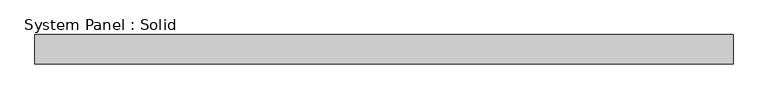
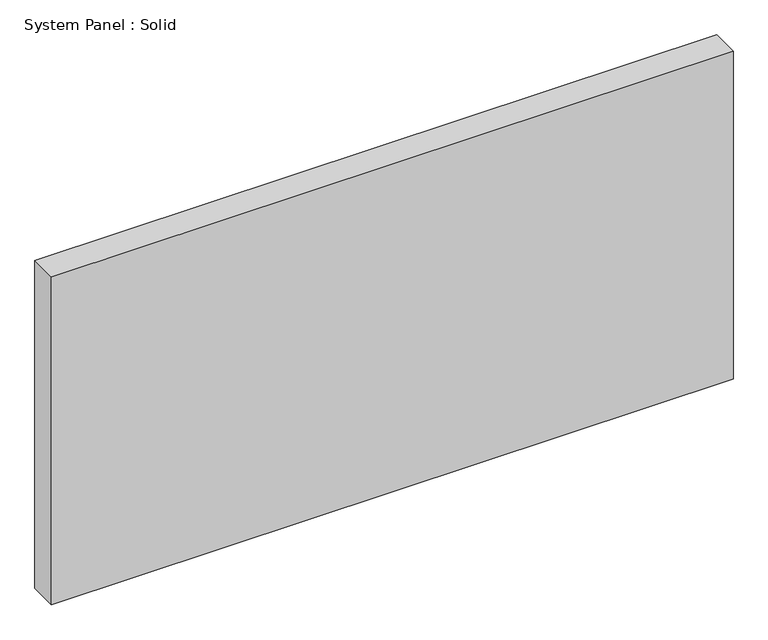
"""IFC4 building model written with IfcOpenShell, lengths in millimetres: plate geometry, System Panel : Solid."""

import ifcopenshell
import ifcopenshell.guid

model = None  # the IFC model being written
_history = None  # IfcOwnerHistory: only IFC2X3 demands one
_inside = {}  # id of a spatial element -> (the spatial element, [elements in it])
_under = {}  # id of a project, library or spatial element -> (it, [spatial elements below it])
_declared = {}  # id of a project -> (the project, [libraries it declares])
_typed = {}  # id of a type object -> (the type object, [elements of that type])
_made_of = {}  # id of a material, layer set ... -> (it, [elements and type objects made of it])


def new_model(schema):
    """Start an empty IFC model of exactly this schema.

    Asked for "IFC4X3", IfcOpenShell would pick the latest addendum, in which some entities
    have other attributes; the version numbers below select the first issue.
    IFC2X3 requires an IfcOwnerHistory on every rooted entity: one is made here for all.
    """
    global model, _history
    if schema == "IFC4X3":
        model = ifcopenshell.file(schema_version=(4, 3, 0, 0))
    else:
        model = ifcopenshell.file(schema=schema)
    _inside.clear()
    _under.clear()
    _declared.clear()
    _typed.clear()
    _made_of.clear()
    _history = None
    if model.schema == "IFC2X3":
        org = make("IfcOrganization", Name="unknown")
        user = make(
            "IfcPersonAndOrganization",
            ThePerson=make("IfcPerson", FamilyName="unknown"),
            TheOrganization=org,
        )
        app = make(
            "IfcApplication",
            ApplicationDeveloper=org,
            Version="unknown",
            ApplicationFullName="unknown",
            ApplicationIdentifier="unknown",
        )
        _history = make(
            "IfcOwnerHistory",
            OwningUser=user,
            OwningApplication=app,
            ChangeAction="ADDED",
            CreationDate=0,
        )
    return model


def make(cls, **values):
    """One entity of the class cls with the attributes given. An attribute that is None is left unset."""
    return model.create_entity(
        cls, **{name: value for name, value in values.items() if value is not None}
    )


def rooted(cls, **values):
    """An entity with a GlobalId (a new one), such as an element, a storey or a relation."""
    return make(cls, GlobalId=ifcopenshell.guid.new(), OwnerHistory=_history, **values)


def si_unit(unit_type, name, prefix=None):
    """IfcSIUnit, for example si_unit("LENGTHUNIT", "METRE", prefix="MILLI")."""
    return make("IfcSIUnit", UnitType=unit_type, Prefix=prefix, Name=name)


def assignment(units):
    """IfcUnitAssignment: the units of a project."""
    return None if units is None else make("IfcUnitAssignment", Units=units)


def point(xyz):
    """IfcCartesianPoint."""
    return None if xyz is None else make("IfcCartesianPoint", Coordinates=xyz)


def direction(xyz):
    """IfcDirection."""
    return None if xyz is None else make("IfcDirection", DirectionRatios=xyz)


def frame(location, z_axis=None, x_axis=None):
    """IfcAxis2Placement3D, a coordinate frame: its origin and axes. An axis left out is left unset."""
    return make(
        "IfcAxis2Placement3D",
        Location=point(location),
        Axis=direction(z_axis),
        RefDirection=direction(x_axis),
    )


def origin():
    """The frame at (0, 0, 0) with its axes left unset."""
    return frame((0.0, 0.0, 0.0))


def origin_with_axes():
    """The frame at (0, 0, 0) with the z axis (0, 0, 1) and the x axis (1, 0, 0) written out."""
    return frame((0.0, 0.0, 0.0), z_axis=(0.0, 0.0, 1.0), x_axis=(1.0, 0.0, 0.0))


def place(relative_to, where):
    """IfcLocalPlacement: puts the frame where relative to a parent placement (None: the world)."""
    return make(
        "IfcLocalPlacement", PlacementRelTo=relative_to, RelativePlacement=where
    )


def context(
    kind, dimensions, precision=None, world=None, true_north=None, identifier=None
):
    """IfcGeometricRepresentationContext, for example the 3D "Model" context."""
    return make(
        "IfcGeometricRepresentationContext",
        ContextIdentifier=identifier,
        ContextType=kind,
        CoordinateSpaceDimension=dimensions,
        Precision=precision,
        WorldCoordinateSystem=world,
        TrueNorth=true_north,
    )


def project(units=None, contexts=None):
    """IfcProject with its units and contexts."""
    return rooted(
        "IfcProject",
        Name="project",
        RepresentationContexts=contexts,
        UnitsInContext=assignment(units),
    )


def spatial(cls, under=None, at=None, **own):
    """A site, building, storey or space (cls), placed at a placement, below another one or the project."""
    s = rooted(cls, ObjectPlacement=at, **own)
    if under is not None:
        _under.setdefault(under.id(), (under, []))[1].append(s)
    return s


def polyline(points):
    """IfcPolyline through the points."""
    return make("IfcPolyline", Points=[point(p) for p in points])


def outline(outer, holes=None, kind="AREA"):
    """IfcArbitraryClosedProfileDef: a profile drawn as a closed curve; with holes, ...WithVoids."""
    if holes is None:
        return make("IfcArbitraryClosedProfileDef", ProfileType=kind, OuterCurve=outer)
    return make(
        "IfcArbitraryProfileDefWithVoids",
        ProfileType=kind,
        OuterCurve=outer,
        InnerCurves=holes,
    )


def extrude(swept, where, along, depth):
    """IfcExtrudedAreaSolid: the profile swept, set in the frame where, extruded along a direction by depth."""
    return make(
        "IfcExtrudedAreaSolid",
        SweptArea=swept,
        Position=where,
        ExtrudedDirection=direction(along),
        Depth=depth,
    )


def shape(context_of_items, identifier, shape_type, items):
    """IfcShapeRepresentation: the items that make up one representation, for example the "Body"."""
    return make(
        "IfcShapeRepresentation",
        ContextOfItems=context_of_items,
        RepresentationIdentifier=identifier,
        RepresentationType=shape_type,
        Items=items,
    )


def source(mapping_origin, context_of_items, identifier, shape_type, items):
    """IfcRepresentationMap: a shape defined once, which mapped items show again and again."""
    return make(
        "IfcRepresentationMap",
        MappingOrigin=mapping_origin,
        MappedRepresentation=shape(context_of_items, identifier, shape_type, items),
    )


def transform(
    local_origin,
    x_axis=None,
    y_axis=None,
    z_axis=None,
    scale=None,
    scale2=None,
    scale3=None,
    uniform=True,
):
    """IfcCartesianTransformationOperator3D, or its non-uniform kind. x_axis, y_axis, z_axis: its Axis1, 2, 3."""
    if uniform:
        return make(
            "IfcCartesianTransformationOperator3D",
            Axis1=direction(x_axis),
            Axis2=direction(y_axis),
            LocalOrigin=point(local_origin),
            Scale=scale,
            Axis3=direction(z_axis),
        )
    return make(
        "IfcCartesianTransformationOperator3DnonUniform",
        Axis1=direction(x_axis),
        Axis2=direction(y_axis),
        LocalOrigin=point(local_origin),
        Scale=scale,
        Axis3=direction(z_axis),
        Scale2=scale2,
        Scale3=scale3,
    )


def mapped(mapping_source, mapping_target):
    """IfcMappedItem: shows the shape of a source again, moved by a transform."""
    return make(
        "IfcMappedItem", MappingSource=mapping_source, MappingTarget=mapping_target
    )


def made_of(thing, what):
    """Note that an element or type object is made of a material, layer set ...; save() writes the relation."""
    if what is not None:
        _made_of.setdefault(what.id(), (what, []))[1].append(thing)
    return thing


def element(
    cls,
    number,
    at=None,
    inside=None,
    cuts=None,
    type_object=None,
    material=None,
    context=None,
    identifier="Body",
    shape_type=None,
    held_by="IfcProductDefinitionShape",
    body=None,
    shapes=None,
    **own,
):
    """One element of the class cls, such as IfcWall. Its Tag is "e" and its number.

    at: its placement. inside: the storey or other place that contains it. cuts: it is an
    opening in that element (IfcRelVoidsElement). A single representation is given by context,
    identifier, shape_type and body (its items); several are given by shapes. held_by: the class
    of the entity that holds the representations. save() writes the other relations.
    """
    e = rooted(cls, Tag="e%d" % number, ObjectPlacement=at, **own)
    if body is not None:
        shapes = [shape(context, identifier, shape_type, body)]
    if shapes is not None:
        e.Representation = make(held_by, Representations=shapes)
    if inside is not None:
        _inside.setdefault(inside.id(), (inside, []))[1].append(e)
    if cuts is not None:
        rooted(
            "IfcRelVoidsElement", RelatingBuildingElement=cuts, RelatedOpeningElement=e
        )
    if type_object is not None:
        _typed.setdefault(type_object.id(), (type_object, []))[1].append(e)
    return made_of(e, material)


def aggregate(whole, parts):
    """IfcRelAggregates: a whole, such as a stair, and the parts it consists of."""
    return rooted("IfcRelAggregates", RelatingObject=whole, RelatedObjects=parts)


def save(model, path):
    """Write the relations noted so far, then the file.

    IfcRelAggregates (storeys below a building ...), IfcRelContainedInSpatialStructure (elements
    in a storey), IfcRelDefinesByType, IfcRelAssociatesMaterial and IfcRelDeclares: one each for
    every whole, place, type object, material and project.
    """
    for whole, parts in _under.values():
        aggregate(whole, parts)
    for where, things in _inside.values():
        rooted(
            "IfcRelContainedInSpatialStructure",
            RelatedElements=things,
            RelatingStructure=where,
        )
    for kind, things in _typed.values():
        rooted("IfcRelDefinesByType", RelatedObjects=things, RelatingType=kind)
    for what, things in _made_of.values():
        rooted("IfcRelAssociatesMaterial", RelatedObjects=things, RelatingMaterial=what)
    for by, libraries in _declared.values():
        rooted("IfcRelDeclares", RelatingContext=by, RelatedDefinitions=libraries)
    model.write(path)


def system_panel_solid_1c6a8c02(model_context):
    return source(origin(), model_context, "Body", "SweptSolid", [
        extrude(outline(polyline([(712.5000001, -10.5), (-712.5000001, -10.5), (-712.5000001, 49.5), (712.5000001, 49.5), (712.5000001, -10.5)])), origin_with_axes(), (0.0, 0.0, 1.0), 725.0),
    ])


if __name__ == "__main__":
    model = new_model("IFC4")
    model_context = context("Model", 3, world=origin())
    ifc_project = project(units=[si_unit("LENGTHUNIT", "METRE", prefix="MILLI")], contexts=[model_context])
    site = spatial("IfcSite", under=ifc_project)
    building = spatial("IfcBuilding", under=site)
    placement = place(None, origin())
    system_panel_solid_shape = system_panel_solid_1c6a8c02(model_context)
    element("IfcPlate", 1, ObjectType="System Panel : Solid", at=placement, inside=building, context=model_context, shape_type="MappedRepresentation", body=[
        mapped(system_panel_solid_shape, transform((0.0, 0.0, 0.0), x_axis=(1.0, 0.0, 0.0), y_axis=(0.0, 1.0, 0.0), z_axis=(0.0, 0.0, 1.0))),
    ])
    save(model, "model.ifc")

# Revit data of these elements
# Type "System Panel : Solid"
#   Keynote = "H11"
#   Construction Type Id = "MDOOR"
#   Analytic Construction = "Metal"
#   Visual Light Transmittance = 0
#   Solar Heat Gain Coefficient = 0
#   Heat Transfer Coefficient (U) = 3.7021 W/(m²·K)
# Element 1 (IfcPlate, "System Panel : Solid")
#   Materials on its faces: "Default"
# Materials
#   "Default": class "Miscellaneous", colour RGB 127 127 127, transparency 0, Comments = "Rendering appearance not upgraded ", Cost = 0
